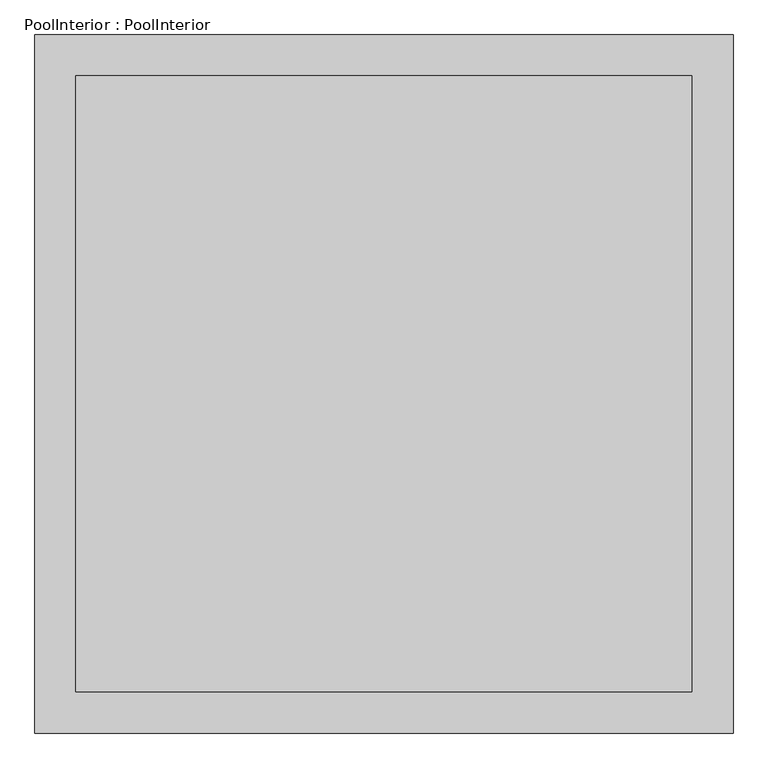
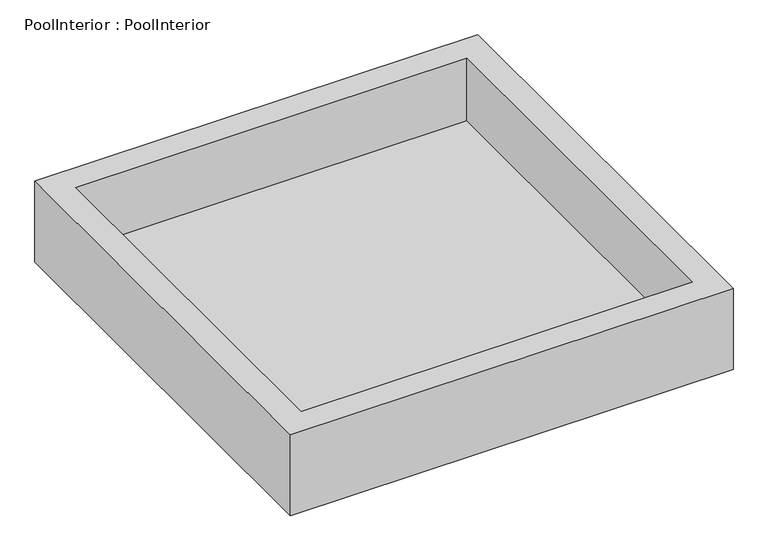
"""IFC4 building model written with IfcOpenShell, lengths in millimetres: proxy geometry, PoolInterior : PoolInterior."""

from ifc_helpers import new_model, si_unit, frame, origin, place, context, project, spatial, polyline, outline, extrude, source, transform, mapped, element, save


def poolinterior_poolinterior_712557d9(model_context):
    return source(origin(), model_context, "Body", "SweptSolid", [
        extrude(outline(polyline([(15021.2046772, 15766.0062171), (15021.2046772, 12766.0062171), (12021.2046772, 12766.0062171), (12021.2046772, 15766.0062171), (15021.2046772, 15766.0062171)])), frame((0.0, 0.0, -557.0896605), z_axis=(0.0, 0.0, 1.0), x_axis=(1.0, 0.0, 0.0)), (0.0, 0.0, 1.0), 149.4528755),
        extrude(outline(polyline([(15221.2046772, 15966.0062171), (15221.2046772, 12566.0062171), (11821.2046772, 12566.0062171), (11821.2046772, 15966.0062171), (15221.2046772, 15966.0062171)]), holes=[polyline([(15021.2046772, 15766.0062171), (12021.2046772, 15766.0062171), (12021.2046772, 12766.0062171), (15021.2046772, 12766.0062171), (15021.2046772, 15766.0062171)])]), frame((0.0, 0.0, -557.0896605), z_axis=(0.0, 0.0, 1.0), x_axis=(1.0, 0.0, 0.0)), (0.0, 0.0, 1.0), 657.0896605),
    ])


if __name__ == "__main__":
    model = new_model("IFC4")
    model_context = context("Model", 3, world=origin())
    ifc_project = project(units=[si_unit("LENGTHUNIT", "METRE", prefix="MILLI")], contexts=[model_context])
    site = spatial("IfcSite", under=ifc_project)
    building = spatial("IfcBuilding", under=site)
    placement = place(None, origin())
    poolinterior_poolinterior_shape = poolinterior_poolinterior_712557d9(model_context)
    element("IfcBuildingElementProxy", 1, Name="PoolInterior : PoolInterior", ObjectType="PoolInterior : PoolInterior", at=placement, inside=building, context=model_context, shape_type="MappedRepresentation", body=[
        mapped(poolinterior_poolinterior_shape, transform((0.0, 0.0, 0.0), x_axis=(1.0, 0.0, 0.0), y_axis=(0.0, 1.0, 0.0), z_axis=(0.0, 0.0, 1.0))),
    ])
    save(model, "model.ifc")

# Revit data of these elements
# Type "PoolInterior : PoolInterior"
#   Height = 0
# Element 1 (IfcBuildingElementProxy, "PoolInterior : PoolInterior")
#   Materials on its faces: "Tile, Porcelain, 4in"
# Materials
#   "Tile, Porcelain, 4in": class "Generic", colour RGB 120 120 120, transparency 0, Description = "Porcelain tile, 4\", white", Cost = 0
